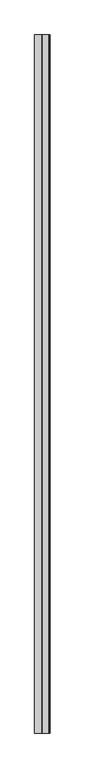
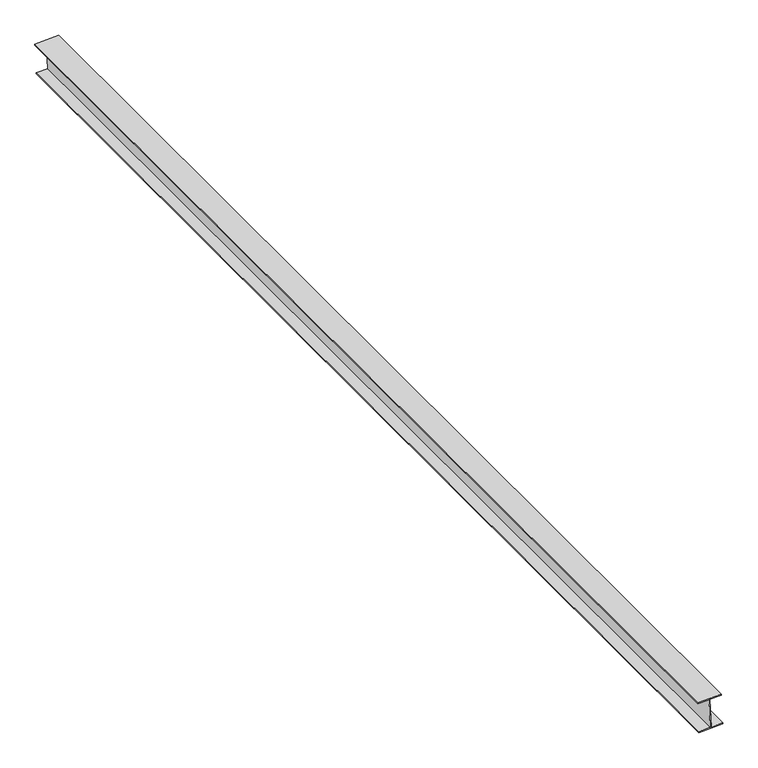
"""IFC4 building model written with IfcOpenShell, lengths in millimetres: proxy geometry, Generic Models 7:Generic Models 1:8:Generic Models 1:8 : Generic Models 7:Generic Models 1:337419:33 : Generic Models 7:Generic Models 1:8:Generic Models 1:8 : Generic Models 7:Generic Models 1:337419:315935."""

import ifcopenshell
import ifcopenshell.guid

model = None  # the IFC model being written
_history = None  # IfcOwnerHistory: only IFC2X3 demands one
_inside = {}  # id of a spatial element -> (the spatial element, [elements in it])
_under = {}  # id of a project, library or spatial element -> (it, [spatial elements below it])
_declared = {}  # id of a project -> (the project, [libraries it declares])
_typed = {}  # id of a type object -> (the type object, [elements of that type])
_made_of = {}  # id of a material, layer set ... -> (it, [elements and type objects made of it])


def new_model(schema):
    """Start an empty IFC model of exactly this schema.

    Asked for "IFC4X3", IfcOpenShell would pick the latest addendum, in which some entities
    have other attributes; the version numbers below select the first issue.
    IFC2X3 requires an IfcOwnerHistory on every rooted entity: one is made here for all.
    """
    global model, _history
    if schema == "IFC4X3":
        model = ifcopenshell.file(schema_version=(4, 3, 0, 0))
    else:
        model = ifcopenshell.file(schema=schema)
    _inside.clear()
    _under.clear()
    _declared.clear()
    _typed.clear()
    _made_of.clear()
    _history = None
    if model.schema == "IFC2X3":
        org = make("IfcOrganization", Name="unknown")
        user = make(
            "IfcPersonAndOrganization",
            ThePerson=make("IfcPerson", FamilyName="unknown"),
            TheOrganization=org,
        )
        app = make(
            "IfcApplication",
            ApplicationDeveloper=org,
            Version="unknown",
            ApplicationFullName="unknown",
            ApplicationIdentifier="unknown",
        )
        _history = make(
            "IfcOwnerHistory",
            OwningUser=user,
            OwningApplication=app,
            ChangeAction="ADDED",
            CreationDate=0,
        )
    return model


def make(cls, **values):
    """One entity of the class cls with the attributes given. An attribute that is None is left unset."""
    return model.create_entity(
        cls, **{name: value for name, value in values.items() if value is not None}
    )


def rooted(cls, **values):
    """An entity with a GlobalId (a new one), such as an element, a storey or a relation."""
    return make(cls, GlobalId=ifcopenshell.guid.new(), OwnerHistory=_history, **values)


def si_unit(unit_type, name, prefix=None):
    """IfcSIUnit, for example si_unit("LENGTHUNIT", "METRE", prefix="MILLI")."""
    return make("IfcSIUnit", UnitType=unit_type, Prefix=prefix, Name=name)


def assignment(units):
    """IfcUnitAssignment: the units of a project."""
    return None if units is None else make("IfcUnitAssignment", Units=units)


def point(xyz):
    """IfcCartesianPoint."""
    return None if xyz is None else make("IfcCartesianPoint", Coordinates=xyz)


def direction(xyz):
    """IfcDirection."""
    return None if xyz is None else make("IfcDirection", DirectionRatios=xyz)


def frame(location, z_axis=None, x_axis=None):
    """IfcAxis2Placement3D, a coordinate frame: its origin and axes. An axis left out is left unset."""
    return make(
        "IfcAxis2Placement3D",
        Location=point(location),
        Axis=direction(z_axis),
        RefDirection=direction(x_axis),
    )


def origin():
    """The frame at (0, 0, 0) with its axes left unset."""
    return frame((0.0, 0.0, 0.0))


def place(relative_to, where):
    """IfcLocalPlacement: puts the frame where relative to a parent placement (None: the world)."""
    return make(
        "IfcLocalPlacement", PlacementRelTo=relative_to, RelativePlacement=where
    )


def context(
    kind, dimensions, precision=None, world=None, true_north=None, identifier=None
):
    """IfcGeometricRepresentationContext, for example the 3D "Model" context."""
    return make(
        "IfcGeometricRepresentationContext",
        ContextIdentifier=identifier,
        ContextType=kind,
        CoordinateSpaceDimension=dimensions,
        Precision=precision,
        WorldCoordinateSystem=world,
        TrueNorth=true_north,
    )


def project(units=None, contexts=None):
    """IfcProject with its units and contexts."""
    return rooted(
        "IfcProject",
        Name="project",
        RepresentationContexts=contexts,
        UnitsInContext=assignment(units),
    )


def spatial(cls, under=None, at=None, **own):
    """A site, building, storey or space (cls), placed at a placement, below another one or the project."""
    s = rooted(cls, ObjectPlacement=at, **own)
    if under is not None:
        _under.setdefault(under.id(), (under, []))[1].append(s)
    return s


def polyline(points):
    """IfcPolyline through the points."""
    return make("IfcPolyline", Points=[point(p) for p in points])


def outline(outer, holes=None, kind="AREA"):
    """IfcArbitraryClosedProfileDef: a profile drawn as a closed curve; with holes, ...WithVoids."""
    if holes is None:
        return make("IfcArbitraryClosedProfileDef", ProfileType=kind, OuterCurve=outer)
    return make(
        "IfcArbitraryProfileDefWithVoids",
        ProfileType=kind,
        OuterCurve=outer,
        InnerCurves=holes,
    )


def extrude(swept, where, along, depth):
    """IfcExtrudedAreaSolid: the profile swept, set in the frame where, extruded along a direction by depth."""
    return make(
        "IfcExtrudedAreaSolid",
        SweptArea=swept,
        Position=where,
        ExtrudedDirection=direction(along),
        Depth=depth,
    )


def shape(context_of_items, identifier, shape_type, items):
    """IfcShapeRepresentation: the items that make up one representation, for example the "Body"."""
    return make(
        "IfcShapeRepresentation",
        ContextOfItems=context_of_items,
        RepresentationIdentifier=identifier,
        RepresentationType=shape_type,
        Items=items,
    )


def source(mapping_origin, context_of_items, identifier, shape_type, items):
    """IfcRepresentationMap: a shape defined once, which mapped items show again and again."""
    return make(
        "IfcRepresentationMap",
        MappingOrigin=mapping_origin,
        MappedRepresentation=shape(context_of_items, identifier, shape_type, items),
    )


def transform(
    local_origin,
    x_axis=None,
    y_axis=None,
    z_axis=None,
    scale=None,
    scale2=None,
    scale3=None,
    uniform=True,
):
    """IfcCartesianTransformationOperator3D, or its non-uniform kind. x_axis, y_axis, z_axis: its Axis1, 2, 3."""
    if uniform:
        return make(
            "IfcCartesianTransformationOperator3D",
            Axis1=direction(x_axis),
            Axis2=direction(y_axis),
            LocalOrigin=point(local_origin),
            Scale=scale,
            Axis3=direction(z_axis),
        )
    return make(
        "IfcCartesianTransformationOperator3DnonUniform",
        Axis1=direction(x_axis),
        Axis2=direction(y_axis),
        LocalOrigin=point(local_origin),
        Scale=scale,
        Axis3=direction(z_axis),
        Scale2=scale2,
        Scale3=scale3,
    )


def mapped(mapping_source, mapping_target):
    """IfcMappedItem: shows the shape of a source again, moved by a transform."""
    return make(
        "IfcMappedItem", MappingSource=mapping_source, MappingTarget=mapping_target
    )


def made_of(thing, what):
    """Note that an element or type object is made of a material, layer set ...; save() writes the relation."""
    if what is not None:
        _made_of.setdefault(what.id(), (what, []))[1].append(thing)
    return thing


def element(
    cls,
    number,
    at=None,
    inside=None,
    cuts=None,
    type_object=None,
    material=None,
    context=None,
    identifier="Body",
    shape_type=None,
    held_by="IfcProductDefinitionShape",
    body=None,
    shapes=None,
    **own,
):
    """One element of the class cls, such as IfcWall. Its Tag is "e" and its number.

    at: its placement. inside: the storey or other place that contains it. cuts: it is an
    opening in that element (IfcRelVoidsElement). A single representation is given by context,
    identifier, shape_type and body (its items); several are given by shapes. held_by: the class
    of the entity that holds the representations. save() writes the other relations.
    """
    e = rooted(cls, Tag="e%d" % number, ObjectPlacement=at, **own)
    if body is not None:
        shapes = [shape(context, identifier, shape_type, body)]
    if shapes is not None:
        e.Representation = make(held_by, Representations=shapes)
    if inside is not None:
        _inside.setdefault(inside.id(), (inside, []))[1].append(e)
    if cuts is not None:
        rooted(
            "IfcRelVoidsElement", RelatingBuildingElement=cuts, RelatedOpeningElement=e
        )
    if type_object is not None:
        _typed.setdefault(type_object.id(), (type_object, []))[1].append(e)
    return made_of(e, material)


def aggregate(whole, parts):
    """IfcRelAggregates: a whole, such as a stair, and the parts it consists of."""
    return rooted("IfcRelAggregates", RelatingObject=whole, RelatedObjects=parts)


def save(model, path):
    """Write the relations noted so far, then the file.

    IfcRelAggregates (storeys below a building ...), IfcRelContainedInSpatialStructure (elements
    in a storey), IfcRelDefinesByType, IfcRelAssociatesMaterial and IfcRelDeclares: one each for
    every whole, place, type object, material and project.
    """
    for whole, parts in _under.values():
        aggregate(whole, parts)
    for where, things in _inside.values():
        rooted(
            "IfcRelContainedInSpatialStructure",
            RelatedElements=things,
            RelatingStructure=where,
        )
    for kind, things in _typed.values():
        rooted("IfcRelDefinesByType", RelatedObjects=things, RelatingType=kind)
    for what, things in _made_of.values():
        rooted("IfcRelAssociatesMaterial", RelatedObjects=things, RelatingMaterial=what)
    for by, libraries in _declared.values():
        rooted("IfcRelDeclares", RelatingContext=by, RelatedDefinitions=libraries)
    model.write(path)


def generic_models_2c7ef85e(model_context):
    return source(origin(), model_context, "Body", "SweptSolid", [
        extrude(outline(polyline([(4024.8136317, 562936.6515986), (4027.7142797, 563009.6189671), (3838.3798209, 563017.1455182), (3835.4784389, 562944.1596862), (3828.6258513, 562944.4320949), (3834.6793776, 563096.7118205), (3841.5319652, 563096.4394118), (3838.621962, 563023.2367072), (4027.9564208, 563015.7101562), (4030.867158, 563088.9313242), (4037.7197456, 563088.6589155), (4031.6662193, 562936.3791899), (4024.8136317, 562936.6515986)])), frame((0.0, -578718.116384, 0.0), z_axis=(0.0, 1.0, 0.0), x_axis=(0.0, 0.0, 1.0)), (0.0, 0.0, 1.0), 7315.2),
    ])


if __name__ == "__main__":
    model = new_model("IFC4")
    model_context = context("Model", 3, world=origin())
    ifc_project = project(units=[si_unit("LENGTHUNIT", "METRE", prefix="MILLI")], contexts=[model_context])
    site = spatial("IfcSite", under=ifc_project)
    building = spatial("IfcBuilding", under=site)
    placement = place(None, origin())
    generic_models_shape = generic_models_2c7ef85e(model_context)
    element("IfcBuildingElementProxy", 1, Name="Generic Models 7:Generic Models 1:8:Generic Models 1:8 : Generic Models 7:Generic Models 1:337419:33 : Generic Models 7:Generic Models 1:8:Generic Models 1:8 : Generic Models 7:Generic Models 1:337419:315935", ObjectType="Generic Models 7:Generic Models 1:8:Generic Models 1:8 : Generic Models 7:Generic Models 1:337419:33 : Generic Models 7:Generic Models 1:8:Generic Models 1:8 : Generic Models 7:Generic Models 1:337419:315935", at=placement, inside=building, context=model_context, shape_type="MappedRepresentation", body=[
        mapped(generic_models_shape, transform((0.0, 0.0, 0.0), x_axis=(1.0, 0.0, 0.0), y_axis=(0.0, 1.0, 0.0), z_axis=(0.0, 0.0, 1.0))),
    ])
    save(model, "model.ifc")

# Revit data of these elements
# Type "Generic Models 7:Generic Models 1:8:Generic Models 1:8 : Generic Models 7:Generic Models 1:337419:33 : Generic Models 7:Generic Models 1:8:Generic Models 1:8 : Generic Models 7:Generic Models 1:337419:315935"
#   NameOverride = "Generic Models 7:Generic Models 1:8:Generic Models 1:8 : Generic Models 7:Generic Models 1:337419:315935"
#   ObjectTypeOverride = "Generic Models 1:8 : Generic Models 7:Generic Models 1:337419"
#   Reference = "Generic Models 1"
#   Tag = "315935"
# Element 1 (IfcBuildingElementProxy, "Generic Models 7:Generic Models 1:8:Generic Models 1:8 : Generic Models 7:Generic Models 1:337419:33 : Generic Models 7:Generic Models 1:8:Generic Models 1:8 : Generic Models 7:Generic Models 1:337419:315935")
#   Materials on its faces: "STRUCTURAL STEEL - SEE STRUCT. DWGS"
# Materials
#   "STRUCTURAL STEEL - SEE STRUCT. DWGS": class "Metal", colour RGB 189 187 185, transparency 0, Description = "Structural steel 50ksi", Cost = 0
